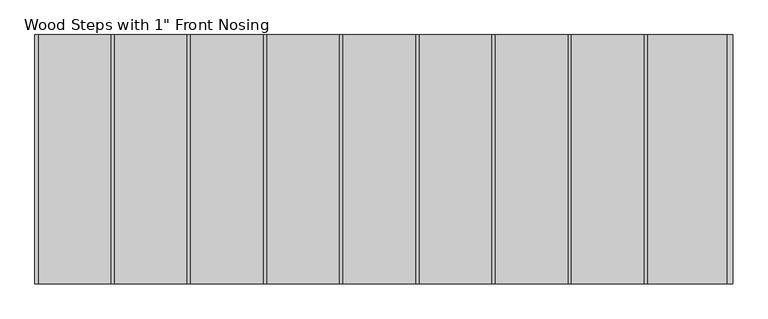
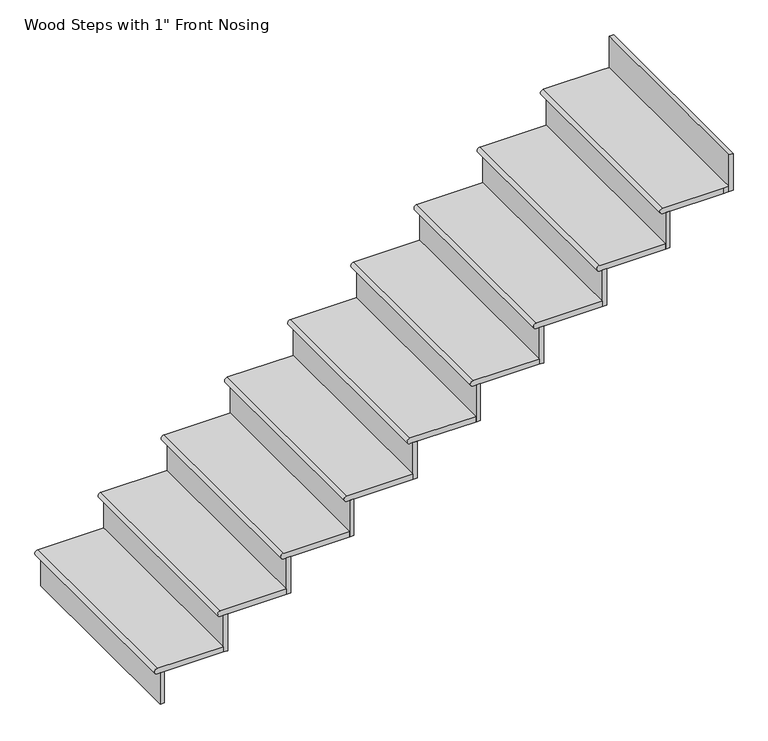
"""IFC4 building model written with IfcOpenShell, lengths in millimetres: stair flight geometry."""

from ifc_helpers import new_model, si_unit, frame, origin, place, context, project, spatial, circle_curve, faceted_brep, source, transform, mapped, element, save
from ifc_brep_helpers import plane_surface, cylinder_surface, advanced_brep


def stair_flight_fa77499c(model_context):
    return source(origin(), model_context, "Body", "SolidModel", [
        advanced_brep(
        [(3725.1741968, -13363.3557429, 2889.25), (3725.1741968, -13363.3557429, 2914.65), (3725.1741968, -12448.9557429, 2914.65), (3725.1741968, -12448.9557429, 2889.25), (4017.2741968, -12448.9557429, 2914.65), (4017.2741968, -13363.3557429, 2914.65), (4017.2741968, -12448.9557429, 2889.25), (4017.2741968, -13363.3557429, 2889.25)],
        [
            (0, 1, circle_curve(frame((3725.1741968, -13363.3557429, 2901.95), z_axis=(0.0, 1.0, 0.0), x_axis=(1.0, 0.0, 0.0)), 12.7)),
            (1, 2),
            (2, 3, circle_curve(frame((3725.1741968, -12448.9557429, 2901.95), z_axis=(0.0, -1.0, 0.0), x_axis=(1.0, 0.0, 0.0)), 12.7)),
            (3, 0),
            (4, 2),
            (1, 5),
            (5, 4),
            (3, 6),
            (6, 7),
            (7, 0),
            (4, 6),
            (7, 5),
        ],
        [
            cylinder_surface(frame((3725.1741968, -13363.3557429, 2901.95), z_axis=(0.0, -1.0, 0.0), x_axis=(1.0, 0.0, 0.0)), 12.7),
            plane_surface(frame((3712.4741968, -12448.9557429, 2914.65), z_axis=(0.0, 0.0, 1.0), x_axis=(-1.0, 0.0, 0.0))),
            plane_surface(frame((3712.4741968, -12448.9557429, 2889.25), z_axis=(0.0, 0.0, -1.0), x_axis=(1.0, 0.0, 0.0))),
            plane_surface(frame((4017.2741968, -12448.9557429, 2914.65), z_axis=(0.0, 1.0, 0.0), x_axis=(0.0, 0.0, -1.0))),
            plane_surface(frame((3725.1741968, -13363.3557429, 2914.65), z_axis=(0.0, -1.0, 0.0), x_axis=(0.0, 0.0, -1.0))),
            plane_surface(frame((4017.2741968, -13363.3557429, 2914.65), z_axis=(1.0, 0.0, 0.0), x_axis=(0.0, 0.0, -1.0))),
        ],
        [
            (0, [[1, 2, 3, 4]]),
            (1, [[5, -2, 6, 7]]),
            (2, [[8, 9, 10, -4]]),
            (3, [[-5, 11, -8, -3]]),
            (4, [[-6, -1, -10, 12]]),
            (5, [[-7, -12, -9, -11]]),
        ],
    ),
        faceted_brep([(3737.8741968, -13363.3557429, 2889.25), (3737.8741968, -13363.3557429, 2743.2), (3756.9241968, -13363.3557429, 2743.2), (3756.9241968, -13363.3557429, 2889.25), (3737.8741968, -12448.9557429, 2889.25), (3756.9241968, -12448.9557429, 2889.25), (3756.9241968, -12448.9557429, 2743.2), (3737.8741968, -12448.9557429, 2743.2)], [[[0, 1, 2, 3]], [[4, 5, 6, 7]], [[1, 0, 4, 7]], [[2, 1, 7, 6]], [[3, 2, 6, 5]], [[0, 3, 5, 4]]]),
        faceted_brep([(4017.2741968, -13363.3557429, 3060.7), (4017.2741968, -13363.3557429, 2889.25), (4036.3241968, -13363.3557429, 2889.25), (4036.3241968, -13363.3557429, 3060.7), (4017.2741968, -12448.9557429, 3060.7), (4036.3241968, -12448.9557429, 3060.7), (4036.3241968, -12448.9557429, 2889.25), (4017.2741968, -12448.9557429, 2889.25)], [[[0, 1, 2, 3]], [[4, 5, 6, 7]], [[1, 0, 4, 7]], [[2, 1, 7, 6]], [[3, 2, 6, 5]], [[0, 3, 5, 4]]]),
        advanced_brep(
        [(4296.6741968, -12448.9557429, 3086.1), (4004.5741968, -12448.9557429, 3086.1), (4004.5741968, -13363.3557429, 3086.1), (4296.6741968, -13363.3557429, 3086.1), (4004.5741968, -12448.9557429, 3060.7), (4296.6741968, -12448.9557429, 3060.7), (4296.6741968, -13363.3557429, 3060.7), (4004.5741968, -13363.3557429, 3060.7)],
        [
            (0, 1),
            (1, 2),
            (2, 3),
            (3, 0),
            (4, 5),
            (5, 6),
            (6, 7),
            (7, 4),
            (0, 5),
            (4, 1, circle_curve(frame((4004.5741968, -12448.9557429, 3073.4), z_axis=(0.0, 1.0, 0.0), x_axis=(1.0, 0.0, 0.0)), 12.7)),
            (2, 7, circle_curve(frame((4004.5741968, -13363.3557429, 3073.4), z_axis=(0.0, -1.0, 0.0), x_axis=(1.0, 0.0, 0.0)), 12.7)),
            (6, 3),
        ],
        [
            plane_surface(frame((3712.4741968, -12448.9557429, 3086.1), z_axis=(0.0, 0.0, 1.0), x_axis=(-1.0, 0.0, 0.0))),
            plane_surface(frame((3712.4741968, -12448.9557429, 3060.7), z_axis=(0.0, 0.0, -1.0), x_axis=(1.0, 0.0, 0.0))),
            plane_surface(frame((4296.6741968, -12448.9557429, 3086.1), z_axis=(0.0, 1.0, 0.0), x_axis=(0.0, 0.0, -1.0))),
            plane_surface(frame((4004.5741968, -13363.3557429, 3086.1), z_axis=(0.0, -1.0, 0.0), x_axis=(0.0, 0.0, -1.0))),
            plane_surface(frame((4296.6741968, -13363.3557429, 3086.1), z_axis=(1.0, 0.0, 0.0), x_axis=(0.0, 0.0, -1.0))),
            cylinder_surface(frame((4004.5741968, -13363.3557429, 3073.4), z_axis=(0.0, -1.0, 0.0), x_axis=(1.0, 0.0, 0.0)), 12.7),
        ],
        [
            (0, [[1, 2, 3, 4]]),
            (1, [[5, 6, 7, 8]]),
            (2, [[-1, 9, -5, 10]]),
            (3, [[-3, 11, -7, 12]]),
            (4, [[-4, -12, -6, -9]]),
            (5, [[-11, -2, -10, -8]]),
        ],
    ),
        faceted_brep([(4296.6741968, -13363.3557429, 3232.15), (4296.6741968, -13363.3557429, 3060.7), (4315.7241968, -13363.3557429, 3060.7), (4315.7241968, -13363.3557429, 3232.15), (4296.6741968, -12448.9557429, 3232.15), (4315.7241968, -12448.9557429, 3232.15), (4315.7241968, -12448.9557429, 3060.7), (4296.6741968, -12448.9557429, 3060.7)], [[[0, 1, 2, 3]], [[4, 5, 6, 7]], [[1, 0, 4, 7]], [[2, 1, 7, 6]], [[3, 2, 6, 5]], [[0, 3, 5, 4]]]),
        advanced_brep(
        [(4576.0741968, -12448.9557429, 3257.55), (4283.9741968, -12448.9557429, 3257.55), (4283.9741968, -13363.3557429, 3257.55), (4576.0741968, -13363.3557429, 3257.55), (4283.9741968, -12448.9557429, 3232.15), (4576.0741968, -12448.9557429, 3232.15), (4576.0741968, -13363.3557429, 3232.15), (4283.9741968, -13363.3557429, 3232.15)],
        [
            (0, 1),
            (1, 2),
            (2, 3),
            (3, 0),
            (4, 5),
            (5, 6),
            (6, 7),
            (7, 4),
            (0, 5),
            (4, 1, circle_curve(frame((4283.9741968, -12448.9557429, 3244.85), z_axis=(0.0, 1.0, 0.0), x_axis=(1.0, 0.0, 0.0)), 12.7)),
            (2, 7, circle_curve(frame((4283.9741968, -13363.3557429, 3244.85), z_axis=(0.0, -1.0, 0.0), x_axis=(1.0, 0.0, 0.0)), 12.7)),
            (6, 3),
        ],
        [
            plane_surface(frame((3991.8741968, -12448.9557429, 3257.55), z_axis=(0.0, 0.0, 1.0), x_axis=(-1.0, 0.0, 0.0))),
            plane_surface(frame((3991.8741968, -12448.9557429, 3232.15), z_axis=(0.0, 0.0, -1.0), x_axis=(1.0, 0.0, 0.0))),
            plane_surface(frame((4576.0741968, -12448.9557429, 3257.55), z_axis=(0.0, 1.0, 0.0), x_axis=(0.0, 0.0, -1.0))),
            plane_surface(frame((4283.9741968, -13363.3557429, 3257.55), z_axis=(0.0, -1.0, 0.0), x_axis=(0.0, 0.0, -1.0))),
            plane_surface(frame((4576.0741968, -13363.3557429, 3257.55), z_axis=(1.0, 0.0, 0.0), x_axis=(0.0, 0.0, -1.0))),
            cylinder_surface(frame((4283.9741968, -13363.3557429, 3244.85), z_axis=(0.0, -1.0, 0.0), x_axis=(1.0, 0.0, 0.0)), 12.7),
        ],
        [
            (0, [[1, 2, 3, 4]]),
            (1, [[5, 6, 7, 8]]),
            (2, [[-1, 9, -5, 10]]),
            (3, [[-3, 11, -7, 12]]),
            (4, [[-4, -12, -6, -9]]),
            (5, [[-11, -2, -10, -8]]),
        ],
    ),
        faceted_brep([(4576.0741968, -13363.3557429, 3403.6), (4576.0741968, -13363.3557429, 3232.15), (4595.1241968, -13363.3557429, 3232.15), (4595.1241968, -13363.3557429, 3403.6), (4576.0741968, -12448.9557429, 3403.6), (4595.1241968, -12448.9557429, 3403.6), (4595.1241968, -12448.9557429, 3232.15), (4576.0741968, -12448.9557429, 3232.15)], [[[0, 1, 2, 3]], [[4, 5, 6, 7]], [[1, 0, 4, 7]], [[2, 1, 7, 6]], [[3, 2, 6, 5]], [[0, 3, 5, 4]]]),
        advanced_brep(
        [(4855.4741968, -12448.9557429, 3429.0), (4563.3741968, -12448.9557429, 3429.0), (4563.3741968, -13363.3557429, 3429.0), (4855.4741968, -13363.3557429, 3429.0), (4563.3741968, -12448.9557429, 3403.6), (4855.4741968, -12448.9557429, 3403.6), (4855.4741968, -13363.3557429, 3403.6), (4563.3741968, -13363.3557429, 3403.6)],
        [
            (0, 1),
            (1, 2),
            (2, 3),
            (3, 0),
            (4, 5),
            (5, 6),
            (6, 7),
            (7, 4),
            (0, 5),
            (4, 1, circle_curve(frame((4563.3741968, -12448.9557429, 3416.3), z_axis=(0.0, 1.0, 0.0), x_axis=(1.0, 0.0, 0.0)), 12.7)),
            (2, 7, circle_curve(frame((4563.3741968, -13363.3557429, 3416.3), z_axis=(0.0, -1.0, 0.0), x_axis=(1.0, 0.0, 0.0)), 12.7)),
            (6, 3),
        ],
        [
            plane_surface(frame((4271.2741968, -12448.9557429, 3429.0), z_axis=(0.0, 0.0, 1.0), x_axis=(-1.0, 0.0, 0.0))),
            plane_surface(frame((4271.2741968, -12448.9557429, 3403.6), z_axis=(0.0, 0.0, -1.0), x_axis=(1.0, 0.0, 0.0))),
            plane_surface(frame((4855.4741968, -12448.9557429, 3429.0), z_axis=(0.0, 1.0, 0.0), x_axis=(0.0, 0.0, -1.0))),
            plane_surface(frame((4563.3741968, -13363.3557429, 3429.0), z_axis=(0.0, -1.0, 0.0), x_axis=(0.0, 0.0, -1.0))),
            plane_surface(frame((4855.4741968, -13363.3557429, 3429.0), z_axis=(1.0, 0.0, 0.0), x_axis=(0.0, 0.0, -1.0))),
            cylinder_surface(frame((4563.3741968, -13363.3557429, 3416.3), z_axis=(0.0, -1.0, 0.0), x_axis=(1.0, 0.0, 0.0)), 12.7),
        ],
        [
            (0, [[1, 2, 3, 4]]),
            (1, [[5, 6, 7, 8]]),
            (2, [[-1, 9, -5, 10]]),
            (3, [[-3, 11, -7, 12]]),
            (4, [[-4, -12, -6, -9]]),
            (5, [[-11, -2, -10, -8]]),
        ],
    ),
        faceted_brep([(4855.4741968, -13363.3557429, 3575.05), (4855.4741968, -13363.3557429, 3403.6), (4874.5241968, -13363.3557429, 3403.6), (4874.5241968, -13363.3557429, 3575.05), (4855.4741968, -12448.9557429, 3575.05), (4874.5241968, -12448.9557429, 3575.05), (4874.5241968, -12448.9557429, 3403.6), (4855.4741968, -12448.9557429, 3403.6)], [[[0, 1, 2, 3]], [[4, 5, 6, 7]], [[1, 0, 4, 7]], [[2, 1, 7, 6]], [[3, 2, 6, 5]], [[0, 3, 5, 4]]]),
        advanced_brep(
        [(5134.8741968, -12448.9557429, 3600.45), (4842.7741968, -12448.9557429, 3600.45), (4842.7741968, -13363.3557429, 3600.45), (5134.8741968, -13363.3557429, 3600.45), (4842.7741968, -12448.9557429, 3575.05), (5134.8741968, -12448.9557429, 3575.05), (5134.8741968, -13363.3557429, 3575.05), (4842.7741968, -13363.3557429, 3575.05)],
        [
            (0, 1),
            (1, 2),
            (2, 3),
            (3, 0),
            (4, 5),
            (5, 6),
            (6, 7),
            (7, 4),
            (0, 5),
            (4, 1, circle_curve(frame((4842.7741968, -12448.9557429, 3587.75), z_axis=(0.0, 1.0, 0.0), x_axis=(1.0, 0.0, 0.0)), 12.7)),
            (2, 7, circle_curve(frame((4842.7741968, -13363.3557429, 3587.75), z_axis=(0.0, -1.0, 0.0), x_axis=(1.0, 0.0, 0.0)), 12.7)),
            (6, 3),
        ],
        [
            plane_surface(frame((4550.6741968, -12448.9557429, 3600.45), z_axis=(0.0, 0.0, 1.0), x_axis=(-1.0, 0.0, 0.0))),
            plane_surface(frame((4550.6741968, -12448.9557429, 3575.05), z_axis=(0.0, 0.0, -1.0), x_axis=(1.0, 0.0, 0.0))),
            plane_surface(frame((5134.8741968, -12448.9557429, 3600.45), z_axis=(0.0, 1.0, 0.0), x_axis=(0.0, 0.0, -1.0))),
            plane_surface(frame((4842.7741968, -13363.3557429, 3600.45), z_axis=(0.0, -1.0, 0.0), x_axis=(0.0, 0.0, -1.0))),
            plane_surface(frame((5134.8741968, -13363.3557429, 3600.45), z_axis=(1.0, 0.0, 0.0), x_axis=(0.0, 0.0, -1.0))),
            cylinder_surface(frame((4842.7741968, -13363.3557429, 3587.75), z_axis=(0.0, -1.0, 0.0), x_axis=(1.0, 0.0, 0.0)), 12.7),
        ],
        [
            (0, [[1, 2, 3, 4]]),
            (1, [[5, 6, 7, 8]]),
            (2, [[-1, 9, -5, 10]]),
            (3, [[-3, 11, -7, 12]]),
            (4, [[-4, -12, -6, -9]]),
            (5, [[-11, -2, -10, -8]]),
        ],
    ),
        faceted_brep([(5134.8741968, -13363.3557429, 3746.5), (5134.8741968, -13363.3557429, 3575.05), (5153.9241968, -13363.3557429, 3575.05), (5153.9241968, -13363.3557429, 3746.5), (5134.8741968, -12448.9557429, 3746.5), (5153.9241968, -12448.9557429, 3746.5), (5153.9241968, -12448.9557429, 3575.05), (5134.8741968, -12448.9557429, 3575.05)], [[[0, 1, 2, 3]], [[4, 5, 6, 7]], [[1, 0, 4, 7]], [[2, 1, 7, 6]], [[3, 2, 6, 5]], [[0, 3, 5, 4]]]),
        advanced_brep(
        [(5414.2741968, -12448.9557429, 3771.9), (5122.1741968, -12448.9557429, 3771.9), (5122.1741968, -13363.3557429, 3771.9), (5414.2741968, -13363.3557429, 3771.9), (5122.1741968, -12448.9557429, 3746.5), (5414.2741968, -12448.9557429, 3746.5), (5414.2741968, -13363.3557429, 3746.5), (5122.1741968, -13363.3557429, 3746.5)],
        [
            (0, 1),
            (1, 2),
            (2, 3),
            (3, 0),
            (4, 5),
            (5, 6),
            (6, 7),
            (7, 4),
            (0, 5),
            (4, 1, circle_curve(frame((5122.1741968, -12448.9557429, 3759.2), z_axis=(0.0, 1.0, 0.0), x_axis=(1.0, 0.0, 0.0)), 12.7)),
            (2, 7, circle_curve(frame((5122.1741968, -13363.3557429, 3759.2), z_axis=(0.0, -1.0, 0.0), x_axis=(1.0, 0.0, 0.0)), 12.7)),
            (6, 3),
        ],
        [
            plane_surface(frame((4830.0741968, -12448.9557429, 3771.9), z_axis=(0.0, 0.0, 1.0), x_axis=(-1.0, 0.0, 0.0))),
            plane_surface(frame((4830.0741968, -12448.9557429, 3746.5), z_axis=(0.0, 0.0, -1.0), x_axis=(1.0, 0.0, 0.0))),
            plane_surface(frame((5414.2741968, -12448.9557429, 3771.9), z_axis=(0.0, 1.0, 0.0), x_axis=(0.0, 0.0, -1.0))),
            plane_surface(frame((5122.1741968, -13363.3557429, 3771.9), z_axis=(0.0, -1.0, 0.0), x_axis=(0.0, 0.0, -1.0))),
            plane_surface(frame((5414.2741968, -13363.3557429, 3771.9), z_axis=(1.0, 0.0, 0.0), x_axis=(0.0, 0.0, -1.0))),
            cylinder_surface(frame((5122.1741968, -13363.3557429, 3759.2), z_axis=(0.0, -1.0, 0.0), x_axis=(1.0, 0.0, 0.0)), 12.7),
        ],
        [
            (0, [[1, 2, 3, 4]]),
            (1, [[5, 6, 7, 8]]),
            (2, [[-1, 9, -5, 10]]),
            (3, [[-3, 11, -7, 12]]),
            (4, [[-4, -12, -6, -9]]),
            (5, [[-11, -2, -10, -8]]),
        ],
    ),
        faceted_brep([(5414.2741968, -13363.3557429, 3917.95), (5414.2741968, -13363.3557429, 3746.5), (5433.3241968, -13363.3557429, 3746.5), (5433.3241968, -13363.3557429, 3917.95), (5414.2741968, -12448.9557429, 3917.95), (5433.3241968, -12448.9557429, 3917.95), (5433.3241968, -12448.9557429, 3746.5), (5414.2741968, -12448.9557429, 3746.5)], [[[0, 1, 2, 3]], [[4, 5, 6, 7]], [[1, 0, 4, 7]], [[2, 1, 7, 6]], [[3, 2, 6, 5]], [[0, 3, 5, 4]]]),
        advanced_brep(
        [(5693.6741968, -12448.9557429, 3943.35), (5401.5741968, -12448.9557429, 3943.35), (5401.5741968, -13363.3557429, 3943.35), (5693.6741968, -13363.3557429, 3943.35), (5401.5741968, -12448.9557429, 3917.95), (5693.6741968, -12448.9557429, 3917.95), (5693.6741968, -13363.3557429, 3917.95), (5401.5741968, -13363.3557429, 3917.95)],
        [
            (0, 1),
            (1, 2),
            (2, 3),
            (3, 0),
            (4, 5),
            (5, 6),
            (6, 7),
            (7, 4),
            (0, 5),
            (4, 1, circle_curve(frame((5401.5741968, -12448.9557429, 3930.65), z_axis=(0.0, 1.0, 0.0), x_axis=(1.0, 0.0, 0.0)), 12.7)),
            (2, 7, circle_curve(frame((5401.5741968, -13363.3557429, 3930.65), z_axis=(0.0, -1.0, 0.0), x_axis=(1.0, 0.0, 0.0)), 12.7)),
            (6, 3),
        ],
        [
            plane_surface(frame((5109.4741968, -12448.9557429, 3943.35), z_axis=(0.0, 0.0, 1.0), x_axis=(-1.0, 0.0, 0.0))),
            plane_surface(frame((5109.4741968, -12448.9557429, 3917.95), z_axis=(0.0, 0.0, -1.0), x_axis=(1.0, 0.0, 0.0))),
            plane_surface(frame((5693.6741968, -12448.9557429, 3943.35), z_axis=(0.0, 1.0, 0.0), x_axis=(0.0, 0.0, -1.0))),
            plane_surface(frame((5401.5741968, -13363.3557429, 3943.35), z_axis=(0.0, -1.0, 0.0), x_axis=(0.0, 0.0, -1.0))),
            plane_surface(frame((5693.6741968, -13363.3557429, 3943.35), z_axis=(1.0, 0.0, 0.0), x_axis=(0.0, 0.0, -1.0))),
            cylinder_surface(frame((5401.5741968, -13363.3557429, 3930.65), z_axis=(0.0, -1.0, 0.0), x_axis=(1.0, 0.0, 0.0)), 12.7),
        ],
        [
            (0, [[1, 2, 3, 4]]),
            (1, [[5, 6, 7, 8]]),
            (2, [[-1, 9, -5, 10]]),
            (3, [[-3, 11, -7, 12]]),
            (4, [[-4, -12, -6, -9]]),
            (5, [[-11, -2, -10, -8]]),
        ],
    ),
        faceted_brep([(5693.6741968, -13363.3557429, 4089.4), (5693.6741968, -13363.3557429, 3917.95), (5712.7241968, -13363.3557429, 3917.95), (5712.7241968, -13363.3557429, 4089.4), (5693.6741968, -12448.9557429, 4089.4), (5712.7241968, -12448.9557429, 4089.4), (5712.7241968, -12448.9557429, 3917.95), (5693.6741968, -12448.9557429, 3917.95)], [[[0, 1, 2, 3]], [[4, 5, 6, 7]], [[1, 0, 4, 7]], [[2, 1, 7, 6]], [[3, 2, 6, 5]], [[0, 3, 5, 4]]]),
        advanced_brep(
        [(5973.0741968, -12448.9557429, 4114.8), (5680.9741968, -12448.9557429, 4114.8), (5680.9741968, -13363.3557429, 4114.8), (5973.0741968, -13363.3557429, 4114.8), (5680.9741968, -12448.9557429, 4089.4), (5973.0741968, -12448.9557429, 4089.4), (5973.0741968, -13363.3557429, 4089.4), (5680.9741968, -13363.3557429, 4089.4)],
        [
            (0, 1),
            (1, 2),
            (2, 3),
            (3, 0),
            (4, 5),
            (5, 6),
            (6, 7),
            (7, 4),
            (0, 5),
            (4, 1, circle_curve(frame((5680.9741968, -12448.9557429, 4102.1), z_axis=(0.0, 1.0, 0.0), x_axis=(1.0, 0.0, 0.0)), 12.7)),
            (2, 7, circle_curve(frame((5680.9741968, -13363.3557429, 4102.1), z_axis=(0.0, -1.0, 0.0), x_axis=(1.0, 0.0, 0.0)), 12.7)),
            (6, 3),
        ],
        [
            plane_surface(frame((5388.8741968, -12448.9557429, 4114.8), z_axis=(0.0, 0.0, 1.0), x_axis=(-1.0, 0.0, 0.0))),
            plane_surface(frame((5388.8741968, -12448.9557429, 4089.4), z_axis=(0.0, 0.0, -1.0), x_axis=(1.0, 0.0, 0.0))),
            plane_surface(frame((5973.0741968, -12448.9557429, 4114.8), z_axis=(0.0, 1.0, 0.0), x_axis=(0.0, 0.0, -1.0))),
            plane_surface(frame((5680.9741968, -13363.3557429, 4114.8), z_axis=(0.0, -1.0, 0.0), x_axis=(0.0, 0.0, -1.0))),
            plane_surface(frame((5973.0741968, -13363.3557429, 4114.8), z_axis=(1.0, 0.0, 0.0), x_axis=(0.0, 0.0, -1.0))),
            cylinder_surface(frame((5680.9741968, -13363.3557429, 4102.1), z_axis=(0.0, -1.0, 0.0), x_axis=(1.0, 0.0, 0.0)), 12.7),
        ],
        [
            (0, [[1, 2, 3, 4]]),
            (1, [[5, 6, 7, 8]]),
            (2, [[-1, 9, -5, 10]]),
            (3, [[-3, 11, -7, 12]]),
            (4, [[-4, -12, -6, -9]]),
            (5, [[-11, -2, -10, -8]]),
        ],
    ),
        faceted_brep([(6252.4741968, -13363.3557429, 4432.3), (6252.4741968, -13363.3557429, 4260.85), (6271.5241968, -13363.3557429, 4260.85), (6271.5241968, -13363.3557429, 4432.3), (6252.4741968, -12448.9557429, 4432.3), (6271.5241968, -12448.9557429, 4432.3), (6271.5241968, -12448.9557429, 4260.85), (6252.4741968, -12448.9557429, 4260.85)], [[[0, 1, 2, 3]], [[4, 5, 6, 7]], [[1, 0, 4, 7]], [[2, 1, 7, 6]], [[3, 2, 6, 5]], [[0, 3, 5, 4]]]),
        faceted_brep([(5973.0741968, -13363.3557429, 4260.85), (5973.0741968, -13363.3557429, 4089.4), (5992.1241968, -13363.3557429, 4089.4), (5992.1241968, -13363.3557429, 4260.85), (5973.0741968, -12448.9557429, 4260.85), (5992.1241968, -12448.9557429, 4260.85), (5992.1241968, -12448.9557429, 4089.4), (5973.0741968, -12448.9557429, 4089.4)], [[[0, 1, 2, 3]], [[4, 5, 6, 7]], [[1, 0, 4, 7]], [[2, 1, 7, 6]], [[3, 2, 6, 5]], [[0, 3, 5, 4]]]),
        advanced_brep(
        [(6252.4741968, -12448.9557429, 4286.25), (6227.0741968, -12448.9557429, 4286.25), (5960.3741968, -12448.9557429, 4286.25), (5960.3741968, -13363.3557429, 4286.25), (6227.0741968, -13363.3557429, 4286.25), (6252.4741968, -13363.3557429, 4286.25), (6227.0741968, -12448.9557429, 4260.85), (6252.4741968, -12448.9557429, 4260.85), (6252.4741968, -13363.3557429, 4260.85), (6227.0741968, -13363.3557429, 4260.85), (5960.3741968, -13363.3557429, 4260.85), (5960.3741968, -12448.9557429, 4260.85)],
        [
            (0, 1),
            (1, 2),
            (2, 3),
            (3, 4),
            (4, 5),
            (5, 0),
            (6, 7),
            (7, 8),
            (8, 9),
            (9, 10),
            (10, 11),
            (11, 6),
            (0, 7),
            (6, 1),
            (11, 2, circle_curve(frame((5960.3741968, -12448.9557429, 4273.55), z_axis=(0.0, 1.0, 0.0), x_axis=(1.0, 0.0, 0.0)), 12.7)),
            (3, 10, circle_curve(frame((5960.3741968, -13363.3557429, 4273.55), z_axis=(0.0, -1.0, 0.0), x_axis=(1.0, 0.0, 0.0)), 12.7)),
            (9, 4),
            (8, 5),
        ],
        [
            plane_surface(frame((6227.0741968, -12448.9557429, 4286.25), z_axis=(0.0, 0.0, 1.0), x_axis=(-1.0, 0.0, 0.0))),
            plane_surface(frame((6227.0741968, -12448.9557429, 4260.85), z_axis=(0.0, 0.0, -1.0), x_axis=(1.0, 0.0, 0.0))),
            plane_surface(frame((6252.4741968, -12448.9557429, 4286.25), z_axis=(0.0, 1.0, 0.0), x_axis=(0.0, 0.0, -1.0))),
            plane_surface(frame((6227.0741968, -12448.9557429, 4286.25), z_axis=(0.0, 1.0, 0.0), x_axis=(0.0, 0.0, -1.0))),
            plane_surface(frame((5960.3741968, -13363.3557429, 4286.25), z_axis=(0.0, -1.0, 0.0), x_axis=(0.0, 0.0, -1.0))),
            plane_surface(frame((6227.0741968, -13363.3557429, 4286.25), z_axis=(0.0, -1.0, 0.0), x_axis=(0.0, 0.0, -1.0))),
            plane_surface(frame((6252.4741968, -13363.3557429, 4286.25), z_axis=(1.0, 0.0, 0.0), x_axis=(0.0, 0.0, -1.0))),
            cylinder_surface(frame((5960.3741968, -13363.3557429, 4273.55), z_axis=(0.0, -1.0, 0.0), x_axis=(1.0, 0.0, 0.0)), 12.7),
        ],
        [
            (0, [[1, 2, 3, 4, 5, 6]]),
            (1, [[7, 8, 9, 10, 11, 12]]),
            (2, [[-1, 13, -7, 14]]),
            (3, [[-2, -14, -12, 15]]),
            (4, [[-4, 16, -10, 17]]),
            (5, [[-5, -17, -9, 18]]),
            (6, [[-6, -18, -8, -13]]),
            (7, [[-16, -3, -15, -11]]),
        ],
    ),
    ])


if __name__ == "__main__":
    model = new_model("IFC4")
    model_context = context("Model", 3, world=origin())
    ifc_project = project(units=[si_unit("LENGTHUNIT", "METRE", prefix="MILLI")], contexts=[model_context])
    site = spatial("IfcSite", under=ifc_project)
    building = spatial("IfcBuilding", under=site)
    placement = place(None, origin())
    stair_flight_shape = stair_flight_fa77499c(model_context)
    element("IfcStairFlight", 1, ObjectType="Wood Steps with 1\" Front Nosing", at=placement, inside=building, context=model_context, shape_type="MappedRepresentation", body=[
        mapped(stair_flight_shape, transform((0.0, 0.0, 0.0), x_axis=(1.0, 0.0, 0.0), y_axis=(0.0, 1.0, 0.0), z_axis=(0.0, 0.0, 1.0))),
    ])
    save(model, "model.ifc")

# Revit data of these elements
# Element 1 (IfcStairFlight, "Wood Steps with 1\" Front Nosing")
#   Materials on its faces: "Paints and Coatings", "Cherry"
# Materials
#   "Paints and Coatings": class "Paint", colour RGB 244 244 244, transparency 0, Description = "Interior finish", Cost = 0
#   "Cherry": class "Wood", colour RGB 233 182 144, transparency 0, Description = "Prunus Serotina", Cost = 0
